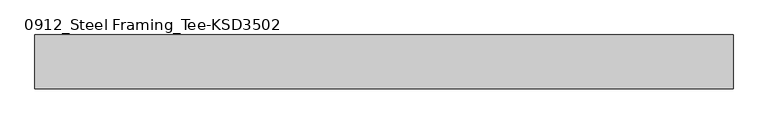
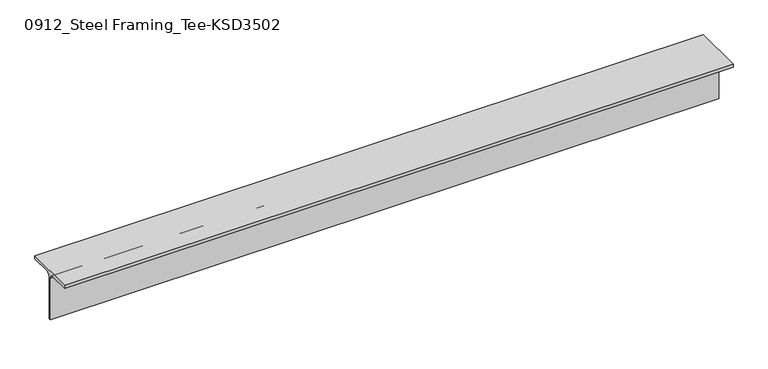
"""IFC4 building model written with IfcOpenShell, lengths in millimetres: member geometry, 0912_Steel Framing_Tee-KSD3502 : H_SB_ASB_CT-150x150x6.5x9."""

from ifc_helpers import new_model, si_unit, point, frame, frame_2d, origin, place, context, project, spatial, polyline, circle_curve, trimmed, segment, composite_curve, outline, extrude, source, transform, mapped, element, save


def member_0912_steel_framing_tee_ksd3502_8de85743(model_context):
    return source(origin(), model_context, "Body", "SweptSolid", [
        extrude(outline(composite_curve([segment(polyline([(75.0, 75.0), (75.0, 66.0), (16.25, 66.0)]), True, "CONTINUOUS"), segment(trimmed(circle_curve(frame_2d((16.25, 53.0)), 13.0), [point((16.25, 66.0))], [point((3.25, 53.0))], True, "CARTESIAN"), True, "CONTINUOUS"), segment(polyline([(3.25, 53.0), (3.25, -75.0), (-3.25, -75.0), (-3.25, 53.0)]), True, "CONTINUOUS"), segment(trimmed(circle_curve(frame_2d((-16.25, 53.0)), 13.0), [point((-3.25, 53.0))], [point((-16.25, 66.0))], True, "CARTESIAN"), True, "CONTINUOUS"), segment(polyline([(-16.25, 66.0), (-75.0, 66.0), (-75.0, 75.0), (75.0, 75.0)]), True, "CONTINUOUS")], self_intersect=False)), frame((-983.95, 0.0, 0.0), z_axis=(1.0, 0.0, 0.0), x_axis=(0.0, 1.0, 0.0)), (0.0, 0.0, 1.0), 1951.2),
    ])


if __name__ == "__main__":
    model = new_model("IFC4")
    model_context = context("Model", 3, world=origin())
    ifc_project = project(units=[si_unit("LENGTHUNIT", "METRE", prefix="MILLI")], contexts=[model_context])
    site = spatial("IfcSite", under=ifc_project)
    building = spatial("IfcBuilding", under=site)
    placement = place(None, origin())
    member_0912_steel_framing_tee_ksd3502_shape = member_0912_steel_framing_tee_ksd3502_8de85743(model_context)
    element("IfcMember", 1, ObjectType="0912_Steel Framing_Tee-KSD3502 : H_SB_ASB_CT-150x150x6.5x9", at=placement, inside=building, context=model_context, shape_type="MappedRepresentation", body=[
        mapped(member_0912_steel_framing_tee_ksd3502_shape, transform((0.0, 0.0, 0.0), x_axis=(1.0, 0.0, 0.0), y_axis=(0.0, 1.0, 0.0), z_axis=(0.0, 0.0, 1.0))),
    ])
    save(model, "model.ifc")

# Revit data of these elements
# Type "0912_Steel Framing_Tee-KSD3502 : H_SB_ASB_CT-150x150x6.5x9"
#   H_WM Code_1 = "S01AA003-00001 | Main Steel Structure Fabrication Work | Shelter/Building | Light Steel - Standard (30KG/M>Weight) | Material: (   )"
#   H_WM Code_2 = "S03AA029-00001 | Main Steel Structure Erection Work | Shelter/Building | Light Steel (30KG/M>Weight) | Material: (   )"
#   H_WM Code_3 = "S01AA010-00001 | Main Steel Structure Fabrication Work | Shelter/Building | Steel Painting/Coating | for Non-Fireproofed Steel Surface, Surface Preparation, Primer, Second & Final Coat | Material: (   )"
#   H_Q'ty Cal Type Tag = "SB-Q2"
#   Width = 15.0 cm
#   Web Thickness = 0.65 cm
#   Web Fillet = 1.3 cm
#   Section Area = 23.39 cm²
#   Perimeter = 0.60 m²/m
#   Nominal Weight = 18.40 kgf/m
#   Height = 15.0 cm
#   Flange Thickness = 0.9 cm
#   Centroid Vertical = 7.5 cm
#   Centroid Horizontal = 7.5 cm
#   Length [instance default] = 1.5000 m
#   Structural Material [instance default] = Steel, 45-345
#   Warping Constant = (empty or 0)
#   Torsional Moment of Inertia = 0
#   Section Name Key = ""
#   Plastic Modulus weak axis = 0
#   Plastic Modulus strong axis = 0
#   Moment of Inertia weak axis = 0
#   Moment of Inertia strong axis = 0
#   Elastic Modulus weak axis = 0
#   Elastic Modulus strong axis = 0
#   Bolt Spacing = 0
#   Assembly Code = ""
# Element 1 (IfcMember, "0912_Steel Framing_Tee-KSD3502 : H_SB_ASB_CT-150x150x6.5x9")
#   Structural Material = none
# Materials
#   "Steel, 45-345": class "Metal", colour RGB 189 187 185, transparency 0, Description = "Steel 345 MPa", Cost = 0
